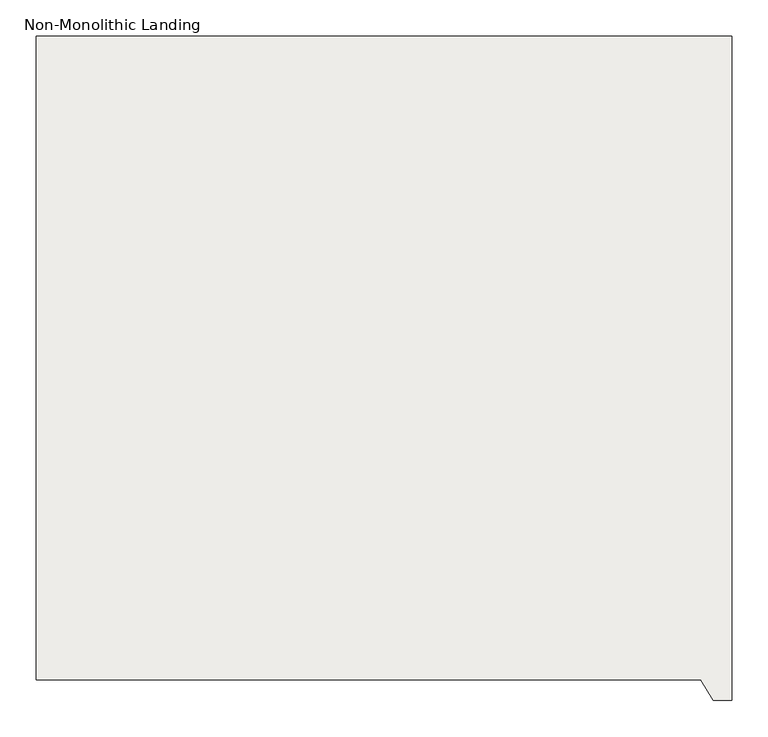
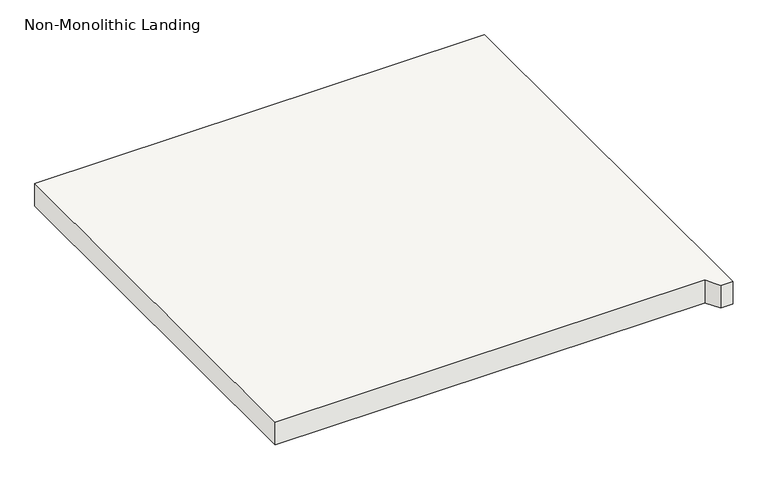
"""IFC4 building model written with IfcOpenShell, lengths in millimetres: slab geometry, Non-Monolithic Landing."""

from ifc_helpers import new_model, si_unit, frame, origin, place, context, project, spatial, polyline, outline, extrude, source, transform, mapped, element, save


def non_monolithic_landing_e25a9e34(model_context):
    return source(origin(), model_context, "Body", "SweptSolid", [
        extrude(outline(polyline([(-9846.4657498, 9677.4676078), (-9846.4657498, 10563.4906648), (-8915.0920821, 10563.4906648), (-8889.6920821, 10563.4906648), (-8889.6920821, 9649.0906648), (-8915.0920821, 9649.0906648), (-8932.0657498, 9677.4676078), (-9846.4657498, 9677.4676078)])), frame((0.0, 0.0, 1457.9451172), z_axis=(0.0, 0.0, 1.0), x_axis=(1.0, 0.0, 0.0)), (0.0, 0.0, 1.0), 50.8),
    ])


if __name__ == "__main__":
    model = new_model("IFC4")
    model_context = context("Model", 3, world=origin())
    ifc_project = project(units=[si_unit("LENGTHUNIT", "METRE", prefix="MILLI")], contexts=[model_context])
    site = spatial("IfcSite", under=ifc_project)
    building = spatial("IfcBuilding", under=site)
    placement = place(None, origin())
    non_monolithic_landing_shape = non_monolithic_landing_e25a9e34(model_context)
    element("IfcSlab", 1, ObjectType="Non-Monolithic Landing", at=placement, inside=building, context=model_context, shape_type="MappedRepresentation", body=[
        mapped(non_monolithic_landing_shape, transform((0.0, 0.0, 0.0), x_axis=(1.0, 0.0, 0.0), y_axis=(0.0, 1.0, 0.0), z_axis=(0.0, 0.0, 1.0))),
    ])
    save(model, "model.ifc")
